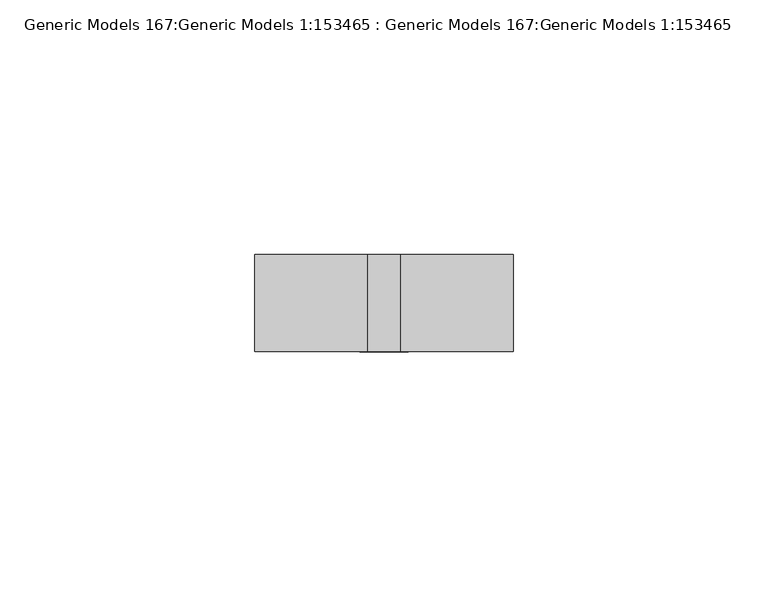
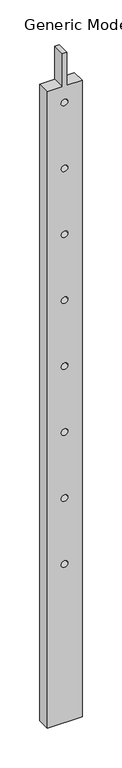
"""IFC4 building model written with IfcOpenShell, lengths in millimetres: proxy geometry, Generic Models 167:Generic Models 1:153465 : Generic Models 167:Generic Models 1:153465."""

from ifc_helpers import new_model, si_unit, point, frame, frame_2d, origin, place, context, project, spatial, polyline, circle_curve, trimmed, segment, composite_curve, outline, extrude, source, transform, mapped, element, save


def generic_models_167_generic_models_1_153465_generic_models_fa3c0082(model_context):
    return source(origin(), model_context, "Body", "SweptSolid", [
        extrude(outline(polyline([(3498.85, -8270.996787), (4479.925, -8270.996787), (4479.925, -8293.221787), (4530.725, -8293.221787), (4530.725, -8299.571787), (4479.925, -8299.571787), (4479.925, -8321.796787), (3498.85, -8321.796787), (3498.85, -8270.996787)]), holes=[composite_curve([segment(trimmed(circle_curve(frame_2d((3743.325, -8296.396787)), 4.7625), [point((3743.325, -8301.159287))], [point((3743.325, -8291.634287))], True, "CARTESIAN"), True, "CONTINUOUS"), segment(trimmed(circle_curve(frame_2d((3743.325, -8296.396787)), 4.7625), [point((3743.325, -8291.634287))], [point((3743.325, -8301.159287))], True, "CARTESIAN"), True, "CONTINUOUS")], self_intersect=False), composite_curve([segment(trimmed(circle_curve(frame_2d((3844.925, -8296.396787)), 4.7625), [point((3844.925, -8301.159287))], [point((3844.925, -8291.634287))], True, "CARTESIAN"), True, "CONTINUOUS"), segment(trimmed(circle_curve(frame_2d((3844.925, -8296.396787)), 4.7625), [point((3844.925, -8291.634287))], [point((3844.925, -8301.159287))], True, "CARTESIAN"), True, "CONTINUOUS")], self_intersect=False), composite_curve([segment(trimmed(circle_curve(frame_2d((3946.525, -8296.396787)), 4.7625), [point((3946.525, -8301.159287))], [point((3946.525, -8291.634287))], True, "CARTESIAN"), True, "CONTINUOUS"), segment(trimmed(circle_curve(frame_2d((3946.525, -8296.396787)), 4.7625), [point((3946.525, -8291.634287))], [point((3946.525, -8301.159287))], True, "CARTESIAN"), True, "CONTINUOUS")], self_intersect=False), composite_curve([segment(trimmed(circle_curve(frame_2d((4048.125, -8296.396787)), 4.7625), [point((4048.125, -8301.159287))], [point((4048.125, -8291.634287))], True, "CARTESIAN"), True, "CONTINUOUS"), segment(trimmed(circle_curve(frame_2d((4048.125, -8296.396787)), 4.7625), [point((4048.125, -8291.634287))], [point((4048.125, -8301.159287))], True, "CARTESIAN"), True, "CONTINUOUS")], self_intersect=False), composite_curve([segment(trimmed(circle_curve(frame_2d((4149.725, -8296.396787)), 4.7625), [point((4149.725, -8301.159287))], [point((4149.725, -8291.634287))], True, "CARTESIAN"), True, "CONTINUOUS"), segment(trimmed(circle_curve(frame_2d((4149.725, -8296.396787)), 4.7625), [point((4149.725, -8291.634287))], [point((4149.725, -8301.159287))], True, "CARTESIAN"), True, "CONTINUOUS")], self_intersect=False), composite_curve([segment(trimmed(circle_curve(frame_2d((4251.325, -8296.396787)), 4.7625), [point((4251.325, -8301.159287))], [point((4251.325, -8291.634287))], True, "CARTESIAN"), True, "CONTINUOUS"), segment(trimmed(circle_curve(frame_2d((4251.325, -8296.396787)), 4.7625), [point((4251.325, -8291.634287))], [point((4251.325, -8301.159287))], True, "CARTESIAN"), True, "CONTINUOUS")], self_intersect=False), composite_curve([segment(trimmed(circle_curve(frame_2d((4352.925, -8296.396787)), 4.7625), [point((4352.925, -8301.159287))], [point((4352.925, -8291.634287))], True, "CARTESIAN"), True, "CONTINUOUS"), segment(trimmed(circle_curve(frame_2d((4352.925, -8296.396787)), 4.7625), [point((4352.925, -8291.634287))], [point((4352.925, -8301.159287))], True, "CARTESIAN"), True, "CONTINUOUS")], self_intersect=False), composite_curve([segment(trimmed(circle_curve(frame_2d((4454.525, -8296.396787)), 4.7625), [point((4454.525, -8301.159287))], [point((4454.525, -8291.634287))], True, "CARTESIAN"), True, "CONTINUOUS"), segment(trimmed(circle_curve(frame_2d((4454.525, -8296.396787)), 4.7625), [point((4454.525, -8291.634287))], [point((4454.525, -8301.159287))], True, "CARTESIAN"), True, "CONTINUOUS")], self_intersect=False)]), frame((0.0, 732.7650592, 0.0), z_axis=(0.0, 1.0, 0.0), x_axis=(0.0, 0.0, 1.0)), (0.0, 0.0, 1.0), 19.05),
    ])


if __name__ == "__main__":
    model = new_model("IFC4")
    model_context = context("Model", 3, world=origin())
    ifc_project = project(units=[si_unit("LENGTHUNIT", "METRE", prefix="MILLI")], contexts=[model_context])
    site = spatial("IfcSite", under=ifc_project)
    building = spatial("IfcBuilding", under=site)
    placement = place(None, origin())
    generic_models_167_generic_models_1_153465_generic_models_shape = generic_models_167_generic_models_1_153465_generic_models_fa3c0082(model_context)
    element("IfcBuildingElementProxy", 1, Name="Generic Models 167:Generic Models 1:153465 : Generic Models 167:Generic Models 1:153465", ObjectType="Generic Models 167:Generic Models 1:153465 : Generic Models 167:Generic Models 1:153465", at=placement, inside=building, context=model_context, shape_type="MappedRepresentation", body=[
        mapped(generic_models_167_generic_models_1_153465_generic_models_shape, transform((0.0, 0.0, 0.0), x_axis=(1.0, 0.0, 0.0), y_axis=(0.0, 1.0, 0.0), z_axis=(0.0, 0.0, 1.0))),
    ])
    save(model, "model.ifc")

# Revit data of these elements
# Type "Generic Models 167:Generic Models 1:153465 : Generic Models 167:Generic Models 1:153465"
#   NameOverride = "Generic Models 167:Generic Models 1:153465"
#   ObjectTypeOverride = "Generic Models 167:Generic Models 1"
#   Reference = "Generic Models 1"
#   Category = "Generic Models"
#   Tag = "153465"
# Element 1 (IfcBuildingElementProxy, "Generic Models 167:Generic Models 1:153465 : Generic Models 167:Generic Models 1:153465")
#   Materials on its faces: "_3/4\" x 1 1/2\" FLAT STOCK PAINTED STEEL POSTS 13787"
# Materials
#   "_3/4\" x 1 1/2\" FLAT STOCK PAINTED STEEL POSTS 13787": class "Unassigned", colour RGB 233 233 233, transparency 0
